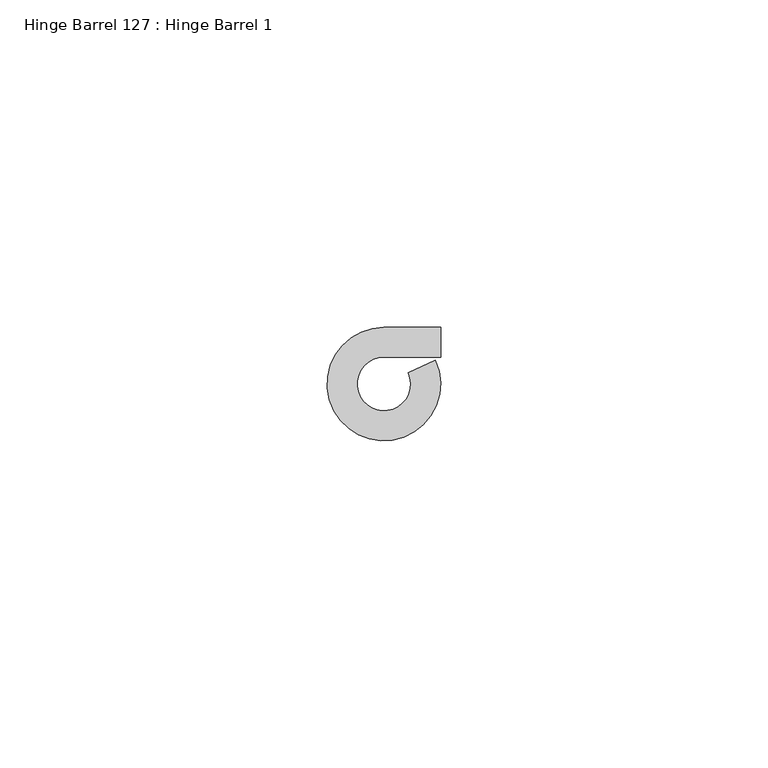
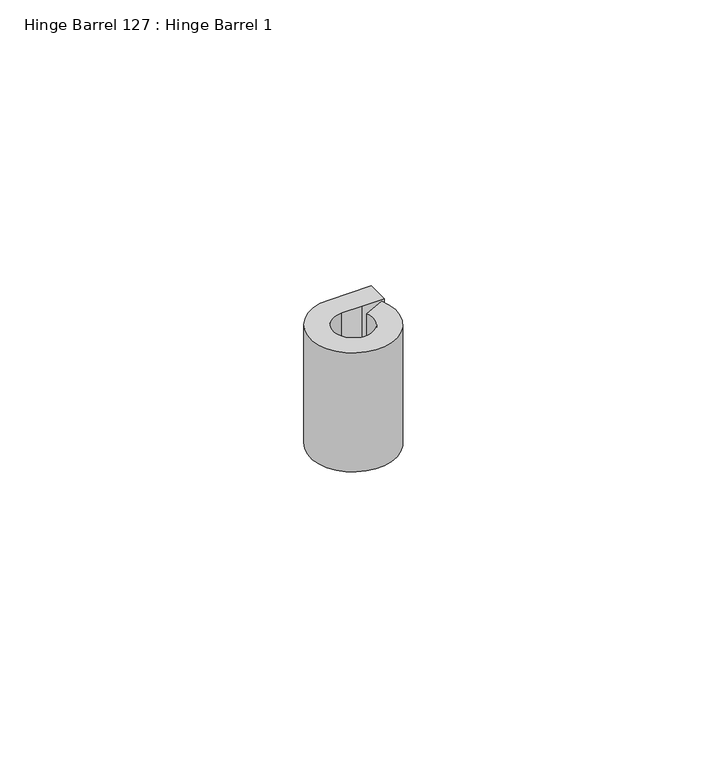
"""IFC4 building model written with IfcOpenShell, lengths in millimetres: proxy geometry, Hinge Barrel 127 : Hinge Barrel 1."""

from ifc_helpers import new_model, si_unit, point, frame, frame_2d, origin, place, context, project, spatial, polyline, circle_curve, trimmed, segment, composite_curve, outline, extrude, source, transform, mapped, element, save


def hinge_barrel_127_hinge_barrel_1_80958469(model_context):
    return source(origin(), model_context, "Body", "SweptSolid", [
        extrude(outline(composite_curve([segment(polyline([(587323.2214739, -536306.2758841), (587319.1320739, -536306.2758841)]), True, "CONTINUOUS"), segment(trimmed(circle_curve(frame_2d((587319.1320739, -536310.3652841)), 4.0894), [point((587319.1320739, -536306.2758841))], [point((587322.8436736, -536308.6485371))], True, "CARTESIAN"), True, "CONTINUOUS"), segment(polyline([(587322.8436736, -536308.6485371), (587326.986084, -536306.7325249)]), True, "CONTINUOUS"), segment(trimmed(circle_curve(frame_2d((587319.1320739, -536310.3652841)), 8.6534625), [point((587326.986084, -536306.7325249))], [point((587319.1320739, -536301.7118216))], False, "CARTESIAN"), True, "CONTINUOUS"), segment(polyline([(587319.1320739, -536301.7118216), (587327.7934739, -536301.7118216), (587327.7934739, -536306.2758841), (587323.2214739, -536306.2758841)]), True, "CONTINUOUS")], self_intersect=False)), frame((0.0, 0.0, 311.15), z_axis=(0.0, 0.0, 1.0), x_axis=(1.0, 0.0, 0.0)), (0.0, 0.0, 1.0), 25.4),
    ])


if __name__ == "__main__":
    model = new_model("IFC4")
    model_context = context("Model", 3, world=origin())
    ifc_project = project(units=[si_unit("LENGTHUNIT", "METRE", prefix="MILLI")], contexts=[model_context])
    site = spatial("IfcSite", under=ifc_project)
    building = spatial("IfcBuilding", under=site)
    placement = place(None, origin())
    hinge_barrel_127_hinge_barrel_1_shape = hinge_barrel_127_hinge_barrel_1_80958469(model_context)
    element("IfcBuildingElementProxy", 1, Name="Hinge Barrel 127 : Hinge Barrel 1", ObjectType="Hinge Barrel 127 : Hinge Barrel 1", at=placement, inside=building, context=model_context, shape_type="MappedRepresentation", body=[
        mapped(hinge_barrel_127_hinge_barrel_1_shape, transform((0.0, 0.0, 0.0), x_axis=(1.0, 0.0, 0.0), y_axis=(0.0, 1.0, 0.0), z_axis=(0.0, 0.0, 1.0))),
    ])
    save(model, "model.ifc")

# Revit data of these elements
# Element 1 (IfcBuildingElementProxy, "Hinge Barrel 127 : Hinge Barrel 1")
#   Materials on its faces: "6\"X6\" WELD-ON STL BUTT HINGE"
# Materials
#   "6\"X6\" WELD-ON STL BUTT HINGE": class "Metal", colour RGB 189 187 185, transparency 0, Description = "Carbon steel", Cost = 0
